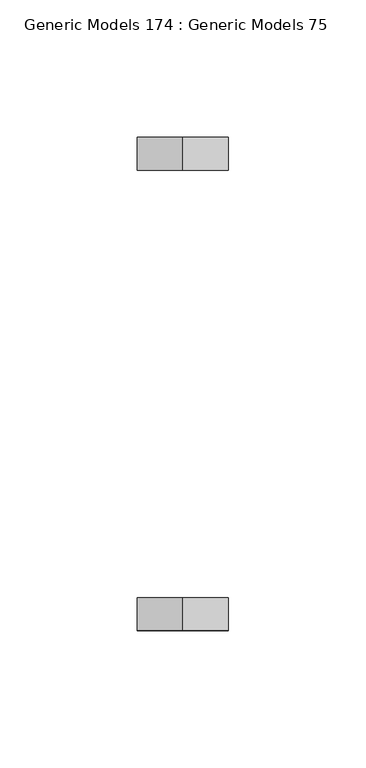
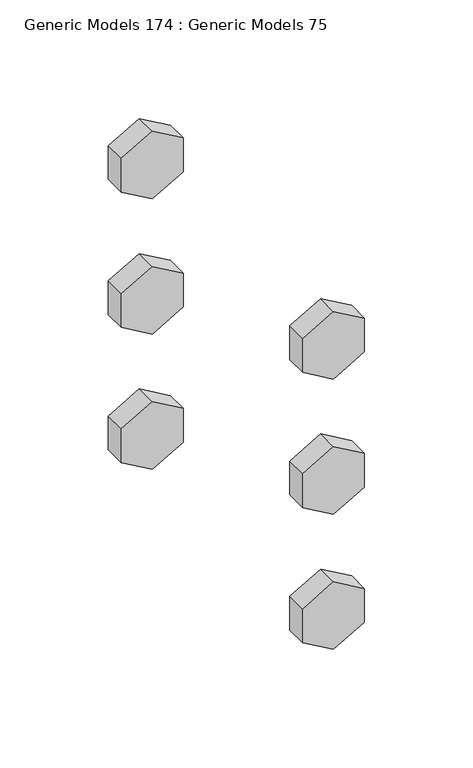
"""IFC4 building model written with IfcOpenShell, lengths in millimetres: proxy geometry, Generic Models 174 : Generic Models 75."""

from ifc_helpers import new_model, si_unit, frame, origin, place, context, project, spatial, polyline, outline, extrude, source, transform, mapped, element, save


def generic_models_174_generic_models_75_1d0625c2(model_context):
    return source(origin(), model_context, "Body", "SweptSolid", [
        extrude(outline(polyline([(271832.3875, 31689.0368192), (271822.8625, 31705.5346032), (271832.3875, 31722.0323871), (271851.4375, 31722.0323871), (271860.9625, 31705.5346032), (271851.4375, 31689.0368192), (271832.3875, 31689.0368192)])), frame((0.0, 30852.1281612, 0.0), z_axis=(0.0, 1.0, 0.0), x_axis=(0.0, 0.0, 1.0)), (0.0, 0.0, 1.0), 11.90625),
        extrude(outline(polyline([(271756.1875, 31689.0368192), (271746.6625, 31705.5346032), (271756.1875, 31722.0323871), (271775.2375, 31722.0323871), (271784.7625, 31705.5346032), (271775.2375, 31689.0368192), (271756.1875, 31689.0368192)])), frame((0.0, 30852.1281612, 0.0), z_axis=(0.0, 1.0, 0.0), x_axis=(0.0, 0.0, 1.0)), (0.0, 0.0, 1.0), 11.90625),
        extrude(outline(polyline([(271679.9875, 31689.0368192), (271670.4625, 31705.5346032), (271679.9875, 31722.0323871), (271699.0375, 31722.0323871), (271708.5625, 31705.5346032), (271699.0375, 31689.0368192), (271679.9875, 31689.0368192)])), frame((0.0, 30852.1281612, 0.0), z_axis=(0.0, 1.0, 0.0), x_axis=(0.0, 0.0, 1.0)), (0.0, 0.0, 1.0), 11.90625),
        extrude(outline(polyline([(271832.3875, 31689.0368192), (271822.8625, 31705.5346032), (271832.3875, 31722.0323871), (271851.4375, 31722.0323871), (271860.9625, 31705.5346032), (271851.4375, 31689.0368192), (271832.3875, 31689.0368192)])), frame((0.0, 30684.6469112, 0.0), z_axis=(0.0, 1.0, 0.0), x_axis=(0.0, 0.0, 1.0)), (0.0, 0.0, 1.0), 11.90625),
        extrude(outline(polyline([(271756.1875, 31689.0368192), (271746.6625, 31705.5346032), (271756.1875, 31722.0323871), (271775.2375, 31722.0323871), (271784.7625, 31705.5346032), (271775.2375, 31689.0368192), (271756.1875, 31689.0368192)])), frame((0.0, 30684.6469112, 0.0), z_axis=(0.0, 1.0, 0.0), x_axis=(0.0, 0.0, 1.0)), (0.0, 0.0, 1.0), 11.90625),
        extrude(outline(polyline([(271679.9875, 31689.0368192), (271670.4625, 31705.5346032), (271679.9875, 31722.0323871), (271699.0375, 31722.0323871), (271708.5625, 31705.5346032), (271699.0375, 31689.0368192), (271679.9875, 31689.0368192)])), frame((0.0, 30684.6469112, 0.0), z_axis=(0.0, 1.0, 0.0), x_axis=(0.0, 0.0, 1.0)), (0.0, 0.0, 1.0), 11.90625),
    ])


if __name__ == "__main__":
    model = new_model("IFC4")
    model_context = context("Model", 3, world=origin())
    ifc_project = project(units=[si_unit("LENGTHUNIT", "METRE", prefix="MILLI")], contexts=[model_context])
    site = spatial("IfcSite", under=ifc_project)
    building = spatial("IfcBuilding", under=site)
    placement = place(None, origin())
    generic_models_174_generic_models_75_shape = generic_models_174_generic_models_75_1d0625c2(model_context)
    element("IfcBuildingElementProxy", 1, Name="Generic Models 174 : Generic Models 75", ObjectType="Generic Models 174 : Generic Models 75", at=placement, inside=building, context=model_context, shape_type="MappedRepresentation", body=[
        mapped(generic_models_174_generic_models_75_shape, transform((0.0, 0.0, 0.0), x_axis=(1.0, 0.0, 0.0), y_axis=(0.0, 1.0, 0.0), z_axis=(0.0, 0.0, 1.0))),
    ])
    save(model, "model.ifc")
